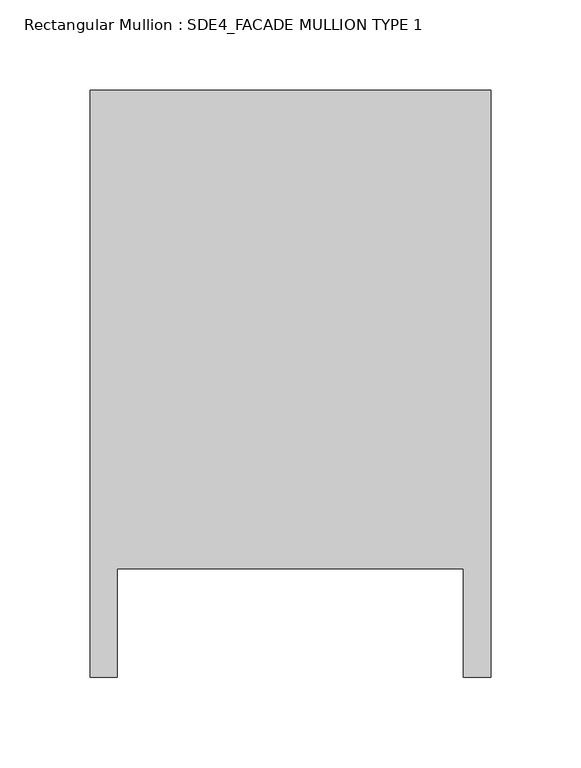
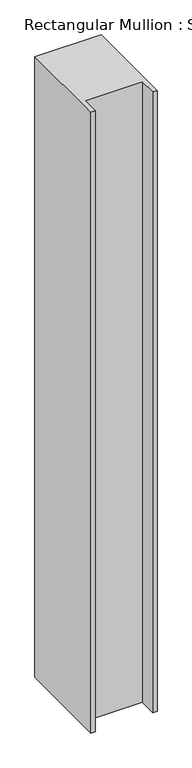
"""IFC4 building model written with IfcOpenShell, lengths in millimetres: member geometry, Rectangular Mullion : SDE4_FACADE MULLION TYPE 1."""

from ifc_helpers import new_model, si_unit, frame, origin, place, context, project, spatial, polyline, outline, extrude, source, transform, mapped, element, save


def rectangular_mullion_sde4_facade_mullion_type_1_f099bba0(model_context):
    return source(origin(), model_context, "Body", "SweptSolid", [
        extrude(outline(polyline([(111.0, 132.5), (111.0, -192.5), (96.0, -192.5), (96.0, -132.5), (-96.0, -132.5), (-96.0, -192.5), (-111.0, -192.5), (-111.0, 132.5), (111.0, 132.5)])), frame((0.0, 0.0, -2200.0), z_axis=(0.0, 0.0, 1.0), x_axis=(1.0, 0.0, 0.0)), (0.0, 0.0, 1.0), 2200.0),
    ])


if __name__ == "__main__":
    model = new_model("IFC4")
    model_context = context("Model", 3, world=origin())
    ifc_project = project(units=[si_unit("LENGTHUNIT", "METRE", prefix="MILLI")], contexts=[model_context])
    site = spatial("IfcSite", under=ifc_project)
    building = spatial("IfcBuilding", under=site)
    placement = place(None, origin())
    rectangular_mullion_sde4_facade_mullion_type_1_shape = rectangular_mullion_sde4_facade_mullion_type_1_f099bba0(model_context)
    element("IfcMember", 1, ObjectType="Rectangular Mullion : SDE4_FACADE MULLION TYPE 1", at=placement, inside=building, context=model_context, shape_type="MappedRepresentation", body=[
        mapped(rectangular_mullion_sde4_facade_mullion_type_1_shape, transform((0.0, 0.0, 0.0), x_axis=(1.0, 0.0, 0.0), y_axis=(0.0, 1.0, 0.0), z_axis=(0.0, 0.0, 1.0))),
    ])
    save(model, "model.ifc")

# Revit data of these elements
# Type "Rectangular Mullion : SDE4_FACADE MULLION TYPE 1"
#   built-in parameter 1007322 = 0.869423 (stored number, unit not read)
#   built-in parameter 1007321 = 0.364173 (stored number, unit not read)
#   built-in parameter 1007320 = 0.364173 (stored number, unit not read)
